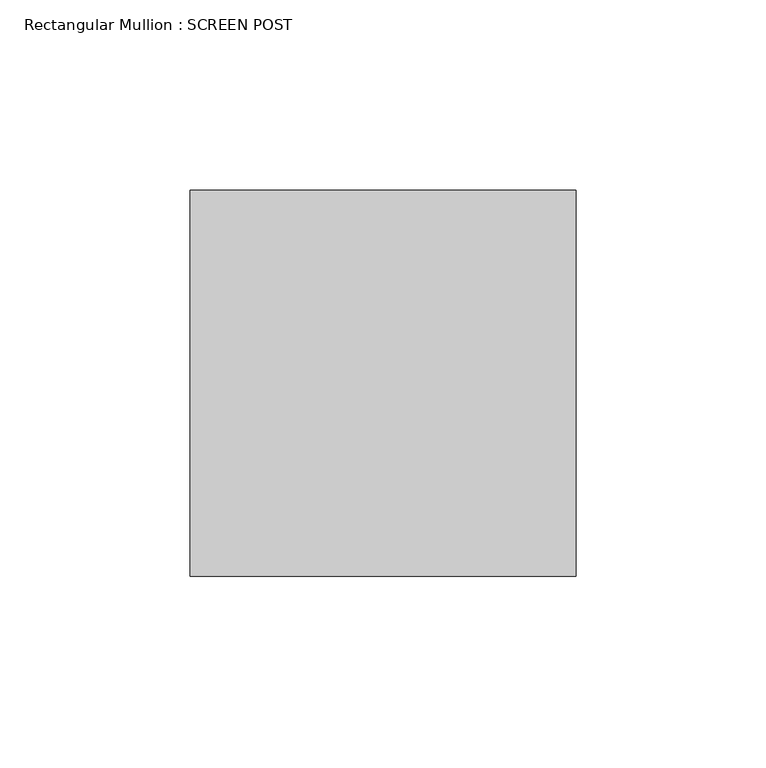
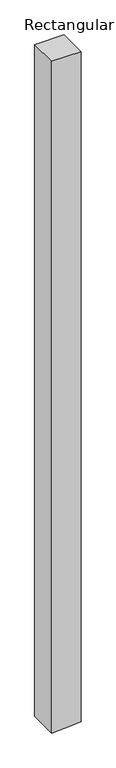
"""IFC4 building model written with IfcOpenShell, lengths in millimetres: member geometry, Rectangular Mullion : SCREEN POST."""

from ifc_helpers import new_model, si_unit, frame, origin, place, context, project, spatial, polyline, outline, extrude, source, transform, mapped, element, save


def rectangular_mullion_screen_post_1bed6209(model_context):
    return source(origin(), model_context, "Body", "SweptSolid", [
        extrude(outline(polyline([(0.0, 50.8), (0.0, -50.8), (-2458.0378572, -50.8), (-2455.2589593, -6.3376339), (-2451.6878572, 50.8), (0.0, 50.8)])), frame((0.0, -50.8, 0.0), z_axis=(0.0, 1.0, 0.0), x_axis=(0.0, 0.0, 1.0)), (0.0, 0.0, 1.0), 101.6),
    ])


if __name__ == "__main__":
    model = new_model("IFC4")
    model_context = context("Model", 3, world=origin())
    ifc_project = project(units=[si_unit("LENGTHUNIT", "METRE", prefix="MILLI")], contexts=[model_context])
    site = spatial("IfcSite", under=ifc_project)
    building = spatial("IfcBuilding", under=site)
    placement = place(None, origin())
    rectangular_mullion_screen_post_shape = rectangular_mullion_screen_post_1bed6209(model_context)
    element("IfcMember", 1, ObjectType="Rectangular Mullion : SCREEN POST", at=placement, inside=building, context=model_context, shape_type="MappedRepresentation", body=[
        mapped(rectangular_mullion_screen_post_shape, transform((0.0, 0.0, 0.0), x_axis=(1.0, 0.0, 0.0), y_axis=(0.0, 1.0, 0.0), z_axis=(0.0, 0.0, 1.0))),
    ])
    save(model, "model.ifc")

# Revit data of these elements
# Type "Rectangular Mullion : SCREEN POST"
#   built-in parameter 1007304 = 0.333333 (stored number, unit not read)
#   built-in parameter 1007301 = 0.166667 (stored number, unit not read)
#   built-in parameter 1007300 = 0.166667 (stored number, unit not read)
# Element 1 (IfcMember, "Rectangular Mullion : SCREEN POST")
#   Materials on its faces: "SCREEN PORCH FRAMING"
# Materials
#   "SCREEN PORCH FRAMING": class "Wood", colour RGB 164 134 123, transparency 0, Description = "Pinus Echinata", Cost = 0
